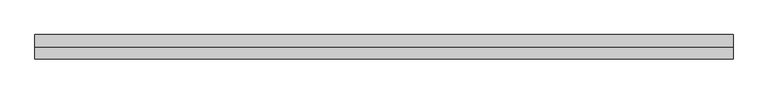
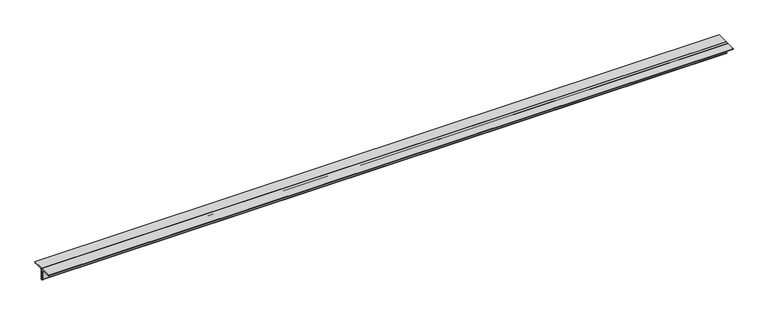
"""IFC4 building model written with IfcOpenShell, lengths in millimetres: beam geometry, 0123_Steel Framing_2Ls-KSD3502 : H_SB_AR_S04_2Ls-130x130x12_VBR2."""

from ifc_helpers import new_model, si_unit, point, frame, frame_2d, origin, place, context, project, spatial, polyline, circle_curve, trimmed, segment, composite_curve, outline, extrude, source, transform, mapped, element, save


def beam_9903f92b(model_context):
    return source(origin(), model_context, "Body", "SweptSolid", [
        extrude(outline(composite_curve([segment(polyline([(0.0, 36.4), (130.0, 36.4)]), True, "CONTINUOUS"), segment(trimmed(circle_curve(frame_2d((118.0, 36.4)), 12.0), [point((130.0, 36.4))], [point((118.0, 24.4))], False, "CARTESIAN"), True, "CONTINUOUS"), segment(polyline([(118.0, 24.4), (24.0, 24.4)]), True, "CONTINUOUS"), segment(trimmed(circle_curve(frame_2d((24.0, 12.4)), 12.0), [point((24.0, 24.4))], [point((12.0, 12.4))], True, "CARTESIAN"), True, "CONTINUOUS"), segment(polyline([(12.0, 12.4), (12.0, -81.6)]), True, "CONTINUOUS"), segment(trimmed(circle_curve(frame_2d((0.0, -81.6)), 12.0), [point((12.0, -81.6))], [point((0.0, -93.6))], False, "CARTESIAN"), True, "CONTINUOUS"), segment(polyline([(0.0, -93.6), (0.0, 36.4)]), True, "CONTINUOUS")], self_intersect=False)), frame((-3854.8431433, 0.0, 0.0), z_axis=(1.0, 0.0, 0.0), x_axis=(0.0, 1.0, 0.0)), (0.0, 0.0, 1.0), 7389.5605416),
        extrude(outline(composite_curve([segment(polyline([(0.0, 36.4), (0.0, -93.6)]), True, "CONTINUOUS"), segment(trimmed(circle_curve(frame_2d((0.0, -81.6)), 12.0), [point((0.0, -93.6))], [point((-12.0, -81.6))], False, "CARTESIAN"), True, "CONTINUOUS"), segment(polyline([(-12.0, -81.6), (-12.0, 12.4)]), True, "CONTINUOUS"), segment(trimmed(circle_curve(frame_2d((-24.0, 12.4)), 12.0), [point((-12.0, 12.4))], [point((-24.0, 24.4))], True, "CARTESIAN"), True, "CONTINUOUS"), segment(polyline([(-24.0, 24.4), (-118.0, 24.4)]), True, "CONTINUOUS"), segment(trimmed(circle_curve(frame_2d((-118.0, 36.4)), 12.0), [point((-118.0, 24.4))], [point((-130.0, 36.4))], False, "CARTESIAN"), True, "CONTINUOUS"), segment(polyline([(-130.0, 36.4), (0.0, 36.4)]), True, "CONTINUOUS")], self_intersect=False)), frame((-3854.8431433, 0.0, 0.0), z_axis=(1.0, 0.0, 0.0), x_axis=(0.0, 1.0, 0.0)), (0.0, 0.0, 1.0), 7389.5605416),
    ])


if __name__ == "__main__":
    model = new_model("IFC4")
    model_context = context("Model", 3, world=origin())
    ifc_project = project(units=[si_unit("LENGTHUNIT", "METRE", prefix="MILLI")], contexts=[model_context])
    site = spatial("IfcSite", under=ifc_project)
    building = spatial("IfcBuilding", under=site)
    placement = place(None, origin())
    beam_shape = beam_9903f92b(model_context)
    element("IfcBeam", 1, ObjectType="0123_Steel Framing_2Ls-KSD3502 : H_SB_AR_S04_2Ls-130x130x12_VBR2", at=placement, inside=building, context=model_context, shape_type="MappedRepresentation", body=[
        mapped(beam_shape, transform((0.0, 0.0, 0.0), x_axis=(1.0, 0.0, 0.0), y_axis=(0.0, 1.0, 0.0), z_axis=(0.0, 0.0, 1.0))),
    ])
    save(model, "model.ifc")

# Revit data of these elements
# Type "0123_Steel Framing_2Ls-KSD3502 : H_SB_AR_S04_2Ls-130x130x12_VBR2"
#   Type Mark = "VBR2"
#   Assembly Code = "B10"
#   Legs = "SLBB"
#   W = 8.97
#   Perimeter = 1.04 m²/m
#   Nominal Weight = 46.80 kgf/m
#   Length [instance default] = 1000 mm
#   Space = 0 mm
#   b = 130 mm
#   d = 130 mm
#   t = 12 mm
#   y = 36.4 mm
#   A = 0.005952 m²
#   Structural Material [instance default] = Steel ASTM A36
# Element 1 (IfcBeam, "0123_Steel Framing_2Ls-KSD3502 : H_SB_AR_S04_2Ls-130x130x12_VBR2")
#   Materials on its faces: "Steel ASTM A36"
# Materials
#   "Steel ASTM A36": class "Metal", colour RGB 199 199 199, transparency 0, Description = "Structural steel, ASTM A36 Grade B, mill finish", Cost = 0
